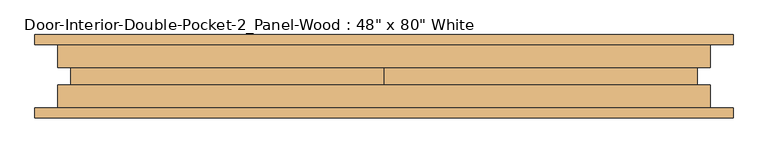
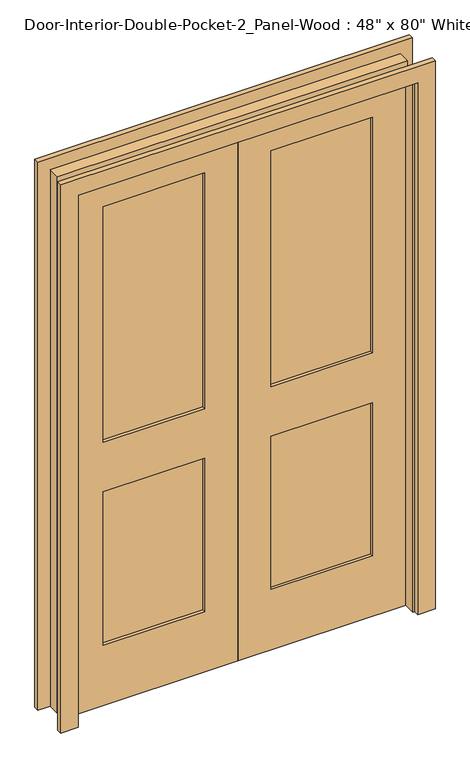
"""IFC4 building model written with IfcOpenShell, lengths in millimetres: door geometry."""

from ifc_helpers import new_model, si_unit, frame, origin, place, context, project, spatial, polyline, outline, extrude, source, transform, mapped, element, save


def door_0fa1dd1a(model_context):
    return source(origin(), model_context, "Body", "SweptSolid", [
        extrude(outline(polyline([(0.0, 615.95), (0.0, 679.45), (2101.85, 679.45), (2101.85, -679.45), (0.0, -679.45), (0.0, -615.95), (2038.35, -615.95), (2038.35, 615.95), (0.0, 615.95)])), frame((0.0, -80.9625, 0.0), z_axis=(0.0, 1.0, 0.0), x_axis=(0.0, 0.0, 1.0)), (0.0, 0.0, 1.0), 19.05),
        extrude(outline(polyline([(0.0, 615.95), (0.0, 679.45), (2101.85, 679.45), (2101.85, -679.45), (0.0, -679.45), (0.0, -615.95), (2038.35, -615.95), (2038.35, 615.95), (0.0, 615.95)])), frame((0.0, 61.9125, 0.0), z_axis=(0.0, 1.0, 0.0), x_axis=(0.0, 0.0, 1.0)), (0.0, 0.0, 1.0), 19.05),
        extrude(outline(polyline([(-120.65, -5.8208333), (-488.95, -5.8208333), (-488.95, 5.8208333), (-120.65, 5.8208333), (-120.65, -5.8208333)])), frame((0.0, 0.0, 1009.65), z_axis=(0.0, 0.0, 1.0), x_axis=(1.0, 0.0, 0.0)), (0.0, 0.0, 1.0), 903.2875),
        extrude(outline(polyline([(-120.65, -5.8208333), (-488.95, -5.8208333), (-488.95, 5.8208333), (-120.65, 5.8208333), (-120.65, -5.8208333)])), frame((0.0, 0.0, 231.775), z_axis=(0.0, 0.0, 1.0), x_axis=(1.0, 0.0, 0.0)), (0.0, 0.0, 1.0), 587.375),
        extrude(outline(polyline([(2032.0, -609.6), (0.0, -609.6), (0.0, 0.0), (2032.0, 0.0), (2032.0, -609.6)]), holes=[polyline([(1912.9375, -488.95), (1912.9375, -120.65), (1009.65, -120.65), (1009.65, -488.95), (1912.9375, -488.95)]), polyline([(819.15, -488.95), (819.15, -120.65), (231.775, -120.65), (231.775, -488.95), (819.15, -488.95)])]), frame((0.0, -17.4625, 0.0), z_axis=(0.0, 1.0, 0.0), x_axis=(0.0, 0.0, 1.0)), (0.0, 0.0, 1.0), 34.925),
        extrude(outline(polyline([(0.0, 635.0), (2057.4, 635.0), (2057.4, -635.0), (0.0, -635.0), (0.0, -609.6), (2032.0, -609.6), (2032.0, 609.6), (0.0, 609.6), (0.0, 635.0)])), frame((0.0, 17.4625, 0.0), z_axis=(0.0, 1.0, 0.0), x_axis=(0.0, 0.0, 1.0)), (0.0, 0.0, 1.0), 44.45),
        extrude(outline(polyline([(0.0, 635.0), (2057.4, 635.0), (2057.4, -635.0), (0.0, -635.0), (0.0, -609.6), (2032.0, -609.6), (2032.0, 609.6), (0.0, 609.6), (0.0, 635.0)])), frame((0.0, -61.9125, 0.0), z_axis=(0.0, 1.0, 0.0), x_axis=(0.0, 0.0, 1.0)), (0.0, 0.0, 1.0), 44.45),
        extrude(outline(polyline([(488.95, -5.8208333), (120.65, -5.8208333), (120.65, 5.8208333), (488.95, 5.8208333), (488.95, -5.8208333)])), frame((0.0, 0.0, 1009.65), z_axis=(0.0, 0.0, 1.0), x_axis=(1.0, 0.0, 0.0)), (0.0, 0.0, 1.0), 903.2875),
        extrude(outline(polyline([(488.95, -5.8208333), (120.65, -5.8208333), (120.65, 5.8208333), (488.95, 5.8208333), (488.95, -5.8208333)])), frame((0.0, 0.0, 231.775), z_axis=(0.0, 0.0, 1.0), x_axis=(1.0, 0.0, 0.0)), (0.0, 0.0, 1.0), 587.375),
        extrude(outline(polyline([(2032.0, 0.0), (0.0, 0.0), (0.0, 609.6), (2032.0, 609.6), (2032.0, 0.0)]), holes=[polyline([(1912.9375, 120.65), (1912.9375, 488.95), (1009.65, 488.95), (1009.65, 120.65), (1912.9375, 120.65)]), polyline([(819.15, 120.65), (819.15, 488.95), (231.775, 488.95), (231.775, 120.65), (819.15, 120.65)])]), frame((0.0, -17.4625, 0.0), z_axis=(0.0, 1.0, 0.0), x_axis=(0.0, 0.0, 1.0)), (0.0, 0.0, 1.0), 34.925),
    ])


if __name__ == "__main__":
    model = new_model("IFC4")
    model_context = context("Model", 3, world=origin())
    ifc_project = project(units=[si_unit("LENGTHUNIT", "METRE", prefix="MILLI")], contexts=[model_context])
    site = spatial("IfcSite", under=ifc_project)
    building = spatial("IfcBuilding", under=site)
    placement = place(None, origin())
    door_shape = door_0fa1dd1a(model_context)
    element("IfcDoor", 1, ObjectType="Door-Interior-Double-Pocket-2_Panel-Wood : 48\" x 80\" White", at=placement, inside=building, context=model_context, shape_type="MappedRepresentation", body=[
        mapped(door_shape, transform((0.0, 0.0, 0.0), x_axis=(1.0, 0.0, 0.0), y_axis=(0.0, 1.0, 0.0), z_axis=(0.0, 0.0, 1.0))),
    ])
    save(model, "model.ifc")

# Revit data of these elements
# Type "Door-Interior-Double-Pocket-2_Panel-Wood : 48\" x 80\" White"
#   Type Mark = "111"
#   COBie.Type.CreatedBy = "doug.wood@us.ibm.com"
#   COBie.Type.CreatedOn = "2016-04-14T02:07:24"
#   COBie.Type.Name = "Doors_Door-Interior-Double-Pocket-2_Panel-Wood_48\" x 80\" White_111"
#   COBie.Type.Category = "23-30 10 00 : Doors"
#   COBie.Type.Description = "Door-Interior-Double-Pocket-2_Panel-Wood_48\" x 80\" White"
#   COBie.Type.Manufacturer = ""
#   COBie.Type.ModelNumber = ""
#   Assembly Code = "C1020300"
#   Analytic Construction = "Wooden"
#   COBie.Type.ReplacementCost = 0
#   Top Rail = 0' - 4 11/16"
#   Thickness = 0' - 1 3/8"
#   Thermal Resistance (R) = 0.455703 (m²·K)/W
#   Stiles = 0' - 4 3/4"
#   Rough Width = 8' - 2"
#   Rough Height = 7' - 0 1/2"
#   Panel Width = 2' - 0"
#   Lock Rail = 0' - 7 1/2"
#   Location [instance default] = 2' - 1"
#   Height = 6' - 8"
#   Width = 4' - 0"
#   Heat Transfer Coefficient (U) = 2.19465 W/(m²·K)
#   Bottom Rail = 0' - 9 1/8"
#   COBie.Type = no
#   Panel Open [instance default] = no
#   Trim Material = Trim - White
#   Panel Material = Door - Frame - White
#   Frame Material = Door - Panel
#   Visual Light Transmittance = 0
#   Solar Heat Gain Coefficient = 0
#   Wall Closure = (empty or 0)
#   Function = (empty or 0)
# Element 1 (IfcDoor, "Door-Interior-Double-Pocket-2_Panel-Wood : 48\" x 80\" White")
#   Materials on its faces: "Door - Frame - White", "Trim - White", "Door - Panel"
# Materials
#   "Trim - White": class "Wood", colour RGB 255 255 255, transparency 0, Cost = 0
#   "Door - Frame - White": class "Miscellaneous", colour RGB 255 255 255, transparency 0, Cost = 0
#   "Door - Panel": class "Wood", colour RGB 255 255 255, transparency 0, Cost = 0
